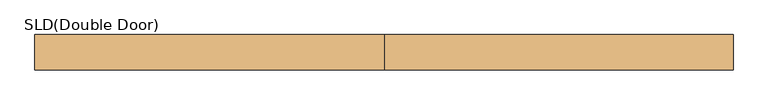
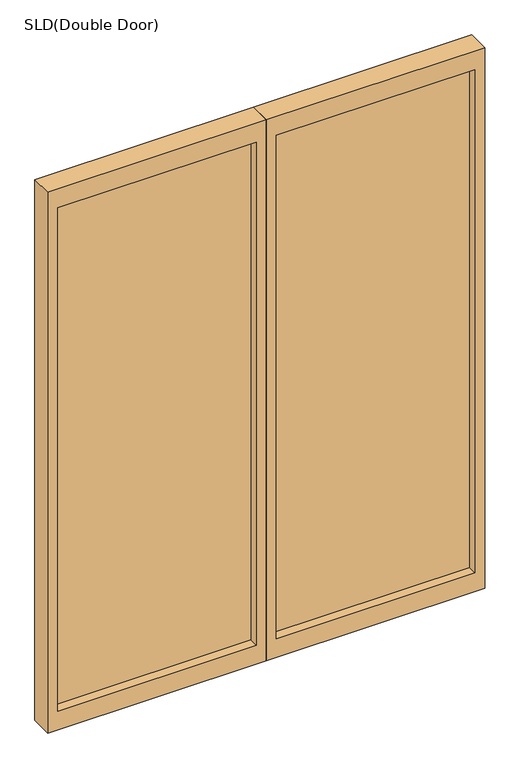
"""IFC4 building model written with IfcOpenShell, lengths in millimetres: door geometry, SLD(Double Door) : H_DR_AR B12_Door_Double_Glass_W2000xH2600_SLD-2."""

from ifc_helpers import new_model, si_unit, frame, origin, place, context, project, spatial, polyline, outline, extrude, source, transform, mapped, element, save


def sld_double_door_31ef1e20(model_context):
    return source(origin(), model_context, "Body", "SweptSolid", [
        extrude(outline(polyline([(-45.0, -151.0), (-945.0, -151.0), (-945.0, -135.0), (-45.0, -135.0), (-45.0, -151.0)])), frame((0.0, 0.0, 90.0), z_axis=(0.0, 0.0, 1.0), x_axis=(1.0, 0.0, 0.0)), (0.0, 0.0, 1.0), 2410.0),
        extrude(outline(polyline([(2590.0, 0.0), (2590.0, -990.0), (0.0, -990.0), (0.0, 0.0), (2590.0, 0.0)]), holes=[polyline([(2500.0, -45.0), (90.0, -45.0), (90.0, -945.0), (2500.0, -945.0), (2500.0, -45.0)])]), frame((0.0, -193.0, 0.0), z_axis=(0.0, 1.0, 0.0), x_axis=(0.0, 0.0, 1.0)), (0.0, 0.0, 1.0), 100.0),
        extrude(outline(polyline([(945.0, -151.0), (45.0, -151.0), (45.0, -135.0), (945.0, -135.0), (945.0, -151.0)])), frame((0.0, 0.0, 90.0), z_axis=(0.0, 0.0, 1.0), x_axis=(1.0, 0.0, 0.0)), (0.0, 0.0, 1.0), 2410.0),
        extrude(outline(polyline([(2590.0, 0.0), (0.0, 0.0), (0.0, 990.0), (2590.0, 990.0), (2590.0, 0.0)]), holes=[polyline([(2500.0, 45.0), (2500.0, 945.0), (90.0, 945.0), (90.0, 45.0), (2500.0, 45.0)])]), frame((0.0, -193.0, 0.0), z_axis=(0.0, 1.0, 0.0), x_axis=(0.0, 0.0, 1.0)), (0.0, 0.0, 1.0), 100.0),
    ])


if __name__ == "__main__":
    model = new_model("IFC4")
    model_context = context("Model", 3, world=origin())
    ifc_project = project(units=[si_unit("LENGTHUNIT", "METRE", prefix="MILLI")], contexts=[model_context])
    site = spatial("IfcSite", under=ifc_project)
    building = spatial("IfcBuilding", under=site)
    placement = place(None, origin())
    sld_double_door_shape = sld_double_door_31ef1e20(model_context)
    element("IfcDoor", 1, ObjectType="SLD(Double Door) : H_DR_AR B12_Door_Double_Glass_W2000xH2600_SLD-2", at=placement, inside=building, context=model_context, shape_type="MappedRepresentation", body=[
        mapped(sld_double_door_shape, transform((0.0, 0.0, 0.0), x_axis=(1.0, 0.0, 0.0), y_axis=(0.0, 1.0, 0.0), z_axis=(0.0, 0.0, 1.0))),
    ])
    save(model, "model.ifc")

# Revit data of these elements
# Type "SLD(Double Door) : H_DR_AR B12_Door_Double_Glass_W2000xH2600_SLD-2"
#   Type Mark = "454"
#   Type Comments = "PD"
#   Analytic Construction = "<None>"
#   Thickness = 45 mm
#   Frame Projection Ext. = 25 mm
#   Frame Projection Int. = 25 mm
#   Frame Width = 75 mm
#   Height = 2600 mm
#   Width = 2000 mm
#   Door Width = 1000 mm
#   Door Frame Thk = 100 mm
#   Center [instance default] = 93 mm
#   Define Thermal Properties by = 1
#   Function = (empty or 0)
#   Wall Closure = (empty or 0)
# Element 1 (IfcDoor, "SLD(Double Door) : H_DR_AR B12_Door_Double_Glass_W2000xH2600_SLD-2")
#   Materials on its faces: "00_Metal_Stainless Steel", "00_Glass_Glass"
# Materials
#   "00_Metal_Stainless Steel": class "Metal", colour RGB 148 148 148, transparency 0, Description = "Steel", Cost = 0
#   "00_Glass_Glass": class "Glass", colour RGB 218 227 224, transparency 0.85, Description = "Glass", Cost = 0, Image = none
